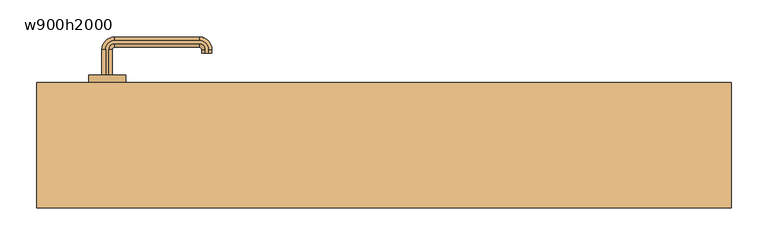
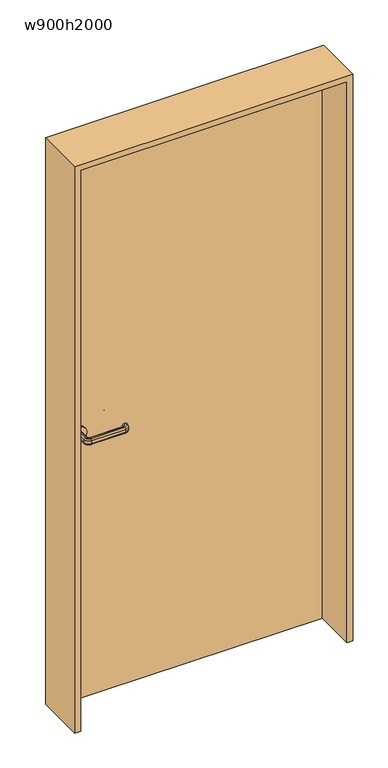
"""IFC4 building model written with IfcOpenShell, lengths in millimetres: door geometry, 片開き : w900h2000."""

from ifc_helpers import new_model, si_unit, point, frame, frame_2d, origin, origin_with_axes, place, context, project, spatial, polyline, circle_curve, ellipse_curve, trimmed, segment, composite_curve, outline, extrude, source, transform, mapped, element, save
from ifc_brep_helpers import plane_surface, cylinder_surface, revolved_surface, advanced_brep


def w900h2000_806be6ba(model_context):
    return source(origin(), model_context, "Body", "SolidModel", [
        advanced_brep(
        [(-377.0, 95.0, 960.0), (-382.0, 95.0, 955.0), (-382.0, 95.0, 945.0477623), (-377.0, 95.0, 940.0477623), (-373.0, 95.0, 940.0477623), (-368.0, 95.0, 945.0477623), (-368.0, 95.0, 955.0), (-373.0, 95.0, 960.0), (-377.0, 130.0, 960.0), (-382.0, 130.0, 955.0), (-382.0, 130.0, 945.0477623), (-377.0, 130.0, 940.0477623), (-365.0, 142.0, 940.0477623), (-250.0, 142.0, 940.0477623), (-238.0, 130.0, 940.0477623), (-238.0, 125.0, 940.0477623), (-242.0, 125.0, 940.0477623), (-242.0, 130.0, 940.0477623), (-250.0, 138.0, 940.0477623), (-365.0, 138.0, 940.0477623), (-373.0, 130.0, 940.0477623), (-368.0, 130.0, 945.0477623), (-368.0, 130.0, 955.0), (-373.0, 130.0, 960.0), (-365.0, 138.0, 960.0), (-250.0, 138.0, 960.0), (-242.0, 130.0, 960.0), (-242.0, 125.0, 960.0), (-238.0, 125.0, 960.0), (-238.0, 130.0, 960.0), (-250.0, 142.0, 960.0), (-365.0, 142.0, 960.0), (-365.0, 147.0, 955.0), (-365.0, 147.0, 945.0477623), (-365.0, 133.0, 945.0477623), (-365.0, 133.0, 955.0), (-250.0, 147.0, 955.0), (-250.0, 147.0, 945.0477623), (-250.0, 133.0, 945.0477623), (-250.0, 133.0, 955.0), (-233.0, 130.0, 955.0), (-233.0, 130.0, 945.0477623), (-247.0, 130.0, 945.0477623), (-247.0, 130.0, 955.0), (-247.0, 125.0, 955.0), (-247.0, 125.0, 945.0477623), (-233.0, 125.0, 945.0477623), (-233.0, 125.0, 955.0)],
        [
            (0, 1, circle_curve(frame((-377.0, 95.0, 955.0), z_axis=(0.0, -1.0, 0.0), x_axis=(-1.0, 0.0, 0.0)), 5.0)),
            (1, 2),
            (2, 3, circle_curve(frame((-377.0, 95.0, 945.0477623), z_axis=(0.0, -1.0, 0.0), x_axis=(-1.0, 0.0, 0.0)), 5.0)),
            (3, 4),
            (4, 5, circle_curve(frame((-373.0, 95.0, 945.0477623), z_axis=(0.0, -1.0, 0.0), x_axis=(-1.0, 0.0, 0.0)), 5.0)),
            (5, 6),
            (6, 7, circle_curve(frame((-373.0, 95.0, 955.0), z_axis=(0.0, -1.0, 0.0), x_axis=(-1.0, 0.0, 0.0)), 5.0)),
            (7, 0),
            (0, 8),
            (8, 9, circle_curve(frame((-377.0, 130.0, 955.0), z_axis=(0.0, -1.0, 0.0), x_axis=(-1.0, 0.0, 0.0)), 5.0)),
            (9, 1),
            (9, 10),
            (10, 2),
            (10, 11, circle_curve(frame((-377.0, 130.0, 945.0477623), z_axis=(0.0, -1.0, 0.0), x_axis=(-1.0, 0.0, 0.0)), 5.0)),
            (11, 3),
            (11, 12, circle_curve(frame((-365.0, 130.0, 940.0477623), z_axis=(0.0, 0.0, -1.0), x_axis=(-1.0, 0.0, 0.0)), 12.0)),
            (12, 13),
            (13, 14, circle_curve(frame((-250.0, 130.0, 940.0477623), z_axis=(0.0, 0.0, -1.0), x_axis=(0.0, 1.0, 0.0)), 12.0)),
            (14, 15),
            (15, 16),
            (16, 17),
            (17, 18, circle_curve(frame((-250.0, 130.0, 940.0477623), z_axis=(0.0, 0.0, 1.0), x_axis=(0.0, 1.0, 0.0)), 8.0)),
            (18, 19),
            (19, 20, circle_curve(frame((-365.0, 130.0, 940.0477623), z_axis=(0.0, 0.0, 1.0), x_axis=(-1.0, 0.0, 0.0)), 8.0)),
            (20, 4),
            (20, 21, circle_curve(frame((-373.0, 130.0, 945.0477623), z_axis=(0.0, -1.0, 0.0), x_axis=(-1.0, 0.0, 0.0)), 5.0)),
            (21, 5),
            (21, 22),
            (22, 6),
            (22, 23, circle_curve(frame((-373.0, 130.0, 955.0), z_axis=(0.0, -1.0, 0.0), x_axis=(-1.0, 0.0, 0.0)), 5.0)),
            (23, 7),
            (23, 24, circle_curve(frame((-365.0, 130.0, 960.0), z_axis=(0.0, 0.0, -1.0), x_axis=(-1.0, 0.0, 0.0)), 8.0)),
            (24, 25),
            (25, 26, circle_curve(frame((-250.0, 130.0, 960.0), z_axis=(0.0, 0.0, -1.0), x_axis=(0.0, 1.0, 0.0)), 8.0)),
            (26, 27),
            (27, 28),
            (28, 29),
            (29, 30, circle_curve(frame((-250.0, 130.0, 960.0), z_axis=(0.0, 0.0, 1.0), x_axis=(0.0, 1.0, 0.0)), 12.0)),
            (30, 31),
            (31, 8, circle_curve(frame((-365.0, 130.0, 960.0), z_axis=(0.0, 0.0, 1.0), x_axis=(-1.0, 0.0, 0.0)), 12.0)),
            (32, 9, circle_curve(frame((-365.0, 130.0, 955.0), z_axis=(0.0, 0.0, 1.0), x_axis=(-1.0, 0.0, 0.0)), 17.0)),
            (31, 32, circle_curve(frame((-365.0, 142.0, 955.0), z_axis=(-1.0, 0.0, 0.0), x_axis=(0.0, 1.0, 0.0)), 5.0)),
            (33, 10, circle_curve(frame((-365.0, 130.0, 945.0477623), z_axis=(0.0, 0.0, 1.0), x_axis=(-1.0, 0.0, 0.0)), 17.0)),
            (32, 33),
            (33, 12, circle_curve(frame((-365.0, 142.0, 945.0477623), z_axis=(-1.0, 0.0, 0.0), x_axis=(0.0, 1.0, 0.0)), 5.0)),
            (34, 21, circle_curve(frame((-365.0, 130.0, 945.0477623), z_axis=(0.0, 0.0, 1.0), x_axis=(-1.0, 0.0, 0.0)), 3.0)),
            (19, 34, circle_curve(frame((-365.0, 138.0, 945.0477623), z_axis=(-1.0, 0.0, 0.0), x_axis=(0.0, 1.0, 0.0)), 5.0)),
            (35, 22, circle_curve(frame((-365.0, 130.0, 955.0), z_axis=(0.0, 0.0, 1.0), x_axis=(-1.0, 0.0, 0.0)), 3.0)),
            (34, 35),
            (35, 24, circle_curve(frame((-365.0, 138.0, 955.0), z_axis=(-1.0, 0.0, 0.0), x_axis=(0.0, 1.0, 0.0)), 5.0)),
            (30, 36, circle_curve(frame((-250.0, 142.0, 955.0), z_axis=(-1.0, 0.0, 0.0), x_axis=(0.0, 1.0, 0.0)), 5.0)),
            (36, 32),
            (36, 37),
            (37, 33),
            (37, 13, circle_curve(frame((-250.0, 142.0, 945.0477623), z_axis=(-1.0, 0.0, 0.0), x_axis=(0.0, 1.0, 0.0)), 5.0)),
            (18, 38, circle_curve(frame((-250.0, 138.0, 945.0477623), z_axis=(-1.0, 0.0, 0.0), x_axis=(0.0, 1.0, 0.0)), 5.0)),
            (38, 34),
            (38, 39),
            (39, 35),
            (39, 25, circle_curve(frame((-250.0, 138.0, 955.0), z_axis=(-1.0, 0.0, 0.0), x_axis=(0.0, 1.0, 0.0)), 5.0)),
            (40, 36, circle_curve(frame((-250.0, 130.0, 955.0), z_axis=(0.0, 0.0, 1.0), x_axis=(0.0, 1.0, 0.0)), 17.0)),
            (29, 40, circle_curve(frame((-238.0, 130.0, 955.0), z_axis=(0.0, 1.0, 0.0), x_axis=(1.0, 0.0, 0.0)), 5.0)),
            (41, 37, circle_curve(frame((-250.0, 130.0, 945.0477623), z_axis=(0.0, 0.0, 1.0), x_axis=(0.0, 1.0, 0.0)), 17.0)),
            (40, 41),
            (41, 14, circle_curve(frame((-238.0, 130.0, 945.0477623), z_axis=(0.0, 1.0, 0.0), x_axis=(1.0, 0.0, 0.0)), 5.0)),
            (42, 38, circle_curve(frame((-250.0, 130.0, 945.0477623), z_axis=(0.0, 0.0, 1.0), x_axis=(0.0, 1.0, 0.0)), 3.0)),
            (17, 42, circle_curve(frame((-242.0, 130.0, 945.0477623), z_axis=(0.0, 1.0, 0.0), x_axis=(1.0, 0.0, 0.0)), 5.0)),
            (43, 39, circle_curve(frame((-250.0, 130.0, 955.0), z_axis=(0.0, 0.0, 1.0), x_axis=(0.0, 1.0, 0.0)), 3.0)),
            (42, 43),
            (43, 26, circle_curve(frame((-242.0, 130.0, 955.0), z_axis=(0.0, 1.0, 0.0), x_axis=(1.0, 0.0, 0.0)), 5.0)),
            (27, 44, circle_curve(frame((-242.0, 125.0, 955.0), z_axis=(0.0, -1.0, 0.0), x_axis=(1.0, 0.0, 0.0)), 5.0)),
            (44, 45),
            (45, 16, circle_curve(frame((-242.0, 125.0, 945.0477623), z_axis=(0.0, -1.0, 0.0), x_axis=(1.0, 0.0, 0.0)), 5.0)),
            (15, 46, circle_curve(frame((-238.0, 125.0, 945.0477623), z_axis=(0.0, -1.0, 0.0), x_axis=(1.0, 0.0, 0.0)), 5.0)),
            (46, 47),
            (47, 28, circle_curve(frame((-238.0, 125.0, 955.0), z_axis=(0.0, -1.0, 0.0), x_axis=(1.0, 0.0, 0.0)), 5.0)),
            (47, 40),
            (46, 41),
            (45, 42),
            (44, 43),
        ],
        [
            plane_surface(frame((-385.198039, 95.0, 950.0), z_axis=(0.0, -1.0, 0.0), x_axis=(0.0, 0.0, 1.0))),
            cylinder_surface(frame((-377.0, 95.0, 955.0), z_axis=(0.0, -1.0, 0.0), x_axis=(-1.0, 0.0, 0.0)), 5.0),
            plane_surface(frame((-382.0, 95.0, 955.0), z_axis=(-1.0, 0.0, 0.0), x_axis=(0.0, 1.0, 0.0))),
            cylinder_surface(frame((-377.0, 95.0, 945.0477623), z_axis=(0.0, -1.0, 0.0), x_axis=(-1.0, 0.0, 0.0)), 5.0),
            plane_surface(frame((-377.0, 95.0, 940.0477623), z_axis=(0.0, 0.0, -1.0), x_axis=(0.0, 1.0, 0.0))),
            cylinder_surface(frame((-373.0, 95.0, 945.0477623), z_axis=(0.0, -1.0, 0.0), x_axis=(-1.0, 0.0, 0.0)), 5.0),
            plane_surface(frame((-368.0, 95.0, 945.0477623), z_axis=(1.0, 0.0, 0.0), x_axis=(0.0, 1.0, 0.0))),
            cylinder_surface(frame((-373.0, 95.0, 955.0), z_axis=(0.0, -1.0, 0.0), x_axis=(-1.0, 0.0, 0.0)), 5.0),
            plane_surface(frame((-373.0, 95.0, 960.0), z_axis=(0.0, 0.0, 1.0), x_axis=(0.0, 1.0, 0.0))),
            revolved_surface(trimmed(ellipse_curve(frame((-377.0, 130.0, 955.0), z_axis=(0.0, -1.0, 0.0), x_axis=(-1.0, 0.0, 0.0)), 5.0, 5.0), [point((-377.0, 130.0, 960.0))], [point((-382.0, 130.0, 955.0))], True, "CARTESIAN"), (-365.0, 130.0, 950.0), (0.0, 0.0, -1.0)),
            cylinder_surface(frame((-365.0, 130.0, 950.0), z_axis=(0.0, 0.0, -1.0), x_axis=(-1.0, 0.0, 0.0)), 17.0),
            revolved_surface(trimmed(ellipse_curve(frame((-377.0, 130.0, 945.0477623), z_axis=(0.0, -1.0, 0.0), x_axis=(-1.0, 0.0, 0.0)), 5.0, 5.0), [point((-382.0, 130.0, 945.0477623))], [point((-377.0, 130.0, 940.0477623))], True, "CARTESIAN"), (-365.0, 130.0, 950.0), (0.0, 0.0, -1.0)),
            revolved_surface(trimmed(ellipse_curve(frame((-373.0, 130.0, 945.0477623), z_axis=(0.0, -1.0, 0.0), x_axis=(-1.0, 0.0, 0.0)), 5.0, 5.0), [point((-373.0, 130.0, 940.0477623))], [point((-368.0, 130.0, 945.0477623))], True, "CARTESIAN"), (-365.0, 130.0, 950.0), (0.0, 0.0, -1.0)),
            revolved_surface(polyline([(-368.0, 130.0, 945.0477623), (-368.0, 130.0, 955.0)]), (-365.0, 130.0, 950.0), (0.0, 0.0, -1.0)),
            revolved_surface(trimmed(ellipse_curve(frame((-373.0, 130.0, 955.0), z_axis=(0.0, -1.0, 0.0), x_axis=(-1.0, 0.0, 0.0)), 5.0, 5.0), [point((-368.0, 130.0, 955.0))], [point((-373.0, 130.0, 960.0))], True, "CARTESIAN"), (-365.0, 130.0, 950.0), (0.0, 0.0, -1.0)),
            cylinder_surface(frame((-365.0, 142.0, 955.0), z_axis=(-1.0, 0.0, 0.0), x_axis=(0.0, 1.0, 0.0)), 5.0),
            plane_surface(frame((-365.0, 147.0, 955.0), z_axis=(0.0, 1.0, 0.0), x_axis=(1.0, 0.0, 0.0))),
            cylinder_surface(frame((-365.0, 142.0, 945.0477623), z_axis=(-1.0, 0.0, 0.0), x_axis=(0.0, 1.0, 0.0)), 5.0),
            cylinder_surface(frame((-365.0, 138.0, 945.0477623), z_axis=(-1.0, 0.0, 0.0), x_axis=(0.0, 1.0, 0.0)), 5.0),
            plane_surface(frame((-365.0, 133.0, 945.0477623), z_axis=(0.0, -1.0, 0.0), x_axis=(1.0, 0.0, 0.0))),
            cylinder_surface(frame((-365.0, 138.0, 955.0), z_axis=(-1.0, 0.0, 0.0), x_axis=(0.0, 1.0, 0.0)), 5.0),
            revolved_surface(trimmed(ellipse_curve(frame((-250.0, 142.0, 955.0), z_axis=(-1.0, 0.0, 0.0), x_axis=(0.0, 1.0, 0.0)), 5.0, 5.0), [point((-250.0, 142.0, 960.0))], [point((-250.0, 147.0, 955.0))], True, "CARTESIAN"), (-250.0, 130.0, 950.0), (0.0, 0.0, -1.0)),
            cylinder_surface(frame((-250.0, 130.0, 950.0), z_axis=(0.0, 0.0, -1.0), x_axis=(0.0, 1.0, 0.0)), 17.0),
            revolved_surface(trimmed(ellipse_curve(frame((-250.0, 142.0, 945.0477623), z_axis=(-1.0, 0.0, 0.0), x_axis=(0.0, 1.0, 0.0)), 5.0, 5.0), [point((-250.0, 147.0, 945.0477623))], [point((-250.0, 142.0, 940.0477623))], True, "CARTESIAN"), (-250.0, 130.0, 950.0), (0.0, 0.0, -1.0)),
            revolved_surface(trimmed(ellipse_curve(frame((-250.0, 138.0, 945.0477623), z_axis=(-1.0, 0.0, 0.0), x_axis=(0.0, 1.0, 0.0)), 5.0, 5.0), [point((-250.0, 138.0, 940.0477623))], [point((-250.0, 133.0, 945.0477623))], True, "CARTESIAN"), (-250.0, 130.0, 950.0), (0.0, 0.0, -1.0)),
            revolved_surface(polyline([(-250.0, 133.0, 945.0477623), (-250.0, 133.0, 955.0)]), (-250.0, 130.0, 950.0), (0.0, 0.0, -1.0)),
            revolved_surface(trimmed(ellipse_curve(frame((-250.0, 138.0, 955.0), z_axis=(-1.0, 0.0, 0.0), x_axis=(0.0, 1.0, 0.0)), 5.0, 5.0), [point((-250.0, 133.0, 955.0))], [point((-250.0, 138.0, 960.0))], True, "CARTESIAN"), (-250.0, 130.0, 950.0), (0.0, 0.0, -1.0)),
            plane_surface(frame((-250.198039, 125.0, 950.0), z_axis=(0.0, -1.0, 0.0), x_axis=(0.0, 0.0, -1.0))),
            cylinder_surface(frame((-238.0, 130.0, 955.0), z_axis=(0.0, 1.0, 0.0), x_axis=(1.0, 0.0, 0.0)), 5.0),
            plane_surface(frame((-233.0, 130.0, 955.0), z_axis=(1.0, 0.0, 0.0), x_axis=(0.0, -1.0, 0.0))),
            cylinder_surface(frame((-238.0, 130.0, 945.0477623), z_axis=(0.0, 1.0, 0.0), x_axis=(1.0, 0.0, 0.0)), 5.0),
            cylinder_surface(frame((-242.0, 130.0, 945.0477623), z_axis=(0.0, 1.0, 0.0), x_axis=(1.0, 0.0, 0.0)), 5.0),
            plane_surface(frame((-247.0, 130.0, 945.0477623), z_axis=(-1.0, 0.0, 0.0), x_axis=(0.0, -1.0, 0.0))),
            cylinder_surface(frame((-242.0, 130.0, 955.0), z_axis=(0.0, 1.0, 0.0), x_axis=(1.0, 0.0, 0.0)), 5.0),
        ],
        [
            (0, [[1, 2, 3, 4, 5, 6, 7, 8]]),
            (1, [[-1, 9, 10, 11]]),
            (2, [[-2, -11, 12, 13]]),
            (3, [[-3, -13, 14, 15]]),
            (4, [[-4, -15, 16, 17, 18, 19, 20, 21, 22, 23, 24, 25]]),
            (5, [[-5, -25, 26, 27]]),
            (6, [[-6, -27, 28, 29]]),
            (7, [[-7, -29, 30, 31]]),
            (8, [[-8, -31, 32, 33, 34, 35, 36, 37, 38, 39, 40, -9]]),
            (9, [[41, -10, -40, 42]]),
            (10, [[43, -12, -41, 44]]),
            (11, [[-16, -14, -43, 45]]),
            (12, [[46, -26, -24, 47]]),
            (13, [[48, -28, -46, 49]]),
            (14, [[-32, -30, -48, 50]]),
            (15, [[-42, -39, 51, 52]]),
            (16, [[-44, -52, 53, 54]]),
            (17, [[-45, -54, 55, -17]]),
            (18, [[-47, -23, 56, 57]]),
            (19, [[-49, -57, 58, 59]]),
            (20, [[-50, -59, 60, -33]]),
            (21, [[61, -51, -38, 62]]),
            (22, [[63, -53, -61, 64]]),
            (23, [[-18, -55, -63, 65]]),
            (24, [[66, -56, -22, 67]]),
            (25, [[68, -58, -66, 69]]),
            (26, [[-34, -60, -68, 70]]),
            (27, [[-36, 71, 72, 73, -20, 74, 75, 76]]),
            (28, [[-62, -37, -76, 77]]),
            (29, [[-64, -77, -75, 78]]),
            (30, [[-65, -78, -74, -19]]),
            (31, [[-67, -21, -73, 79]]),
            (32, [[-69, -79, -72, 80]]),
            (33, [[-70, -80, -71, -35]]),
        ],
    ),
        advanced_brep(
        [(-373.0, 50.0, 940.0), (-377.0, 50.0, 940.0), (-382.0, 50.0, 945.0), (-382.0, 50.0, 955.0), (-377.0, 50.0, 960.0), (-373.0, 50.0, 960.0), (-368.0, 50.0, 955.0), (-368.0, 50.0, 945.0), (-373.0, 15.0, 940.0), (-365.0, 7.0, 940.0), (-250.0, 7.0, 940.0), (-242.0, 15.0, 940.0), (-242.0, 20.0, 940.0), (-238.0, 20.0, 940.0), (-238.0, 15.0, 940.0), (-250.0, 3.0, 940.0), (-365.0, 3.0, 940.0), (-377.0, 15.0, 940.0), (-382.0, 15.0, 945.0), (-382.0, 15.0, 955.0), (-377.0, 15.0, 960.0), (-365.0, 3.0, 960.0), (-250.0, 3.0, 960.0), (-238.0, 15.0, 960.0), (-238.0, 20.0, 960.0), (-242.0, 20.0, 960.0), (-242.0, 15.0, 960.0), (-250.0, 7.0, 960.0), (-365.0, 7.0, 960.0), (-373.0, 15.0, 960.0), (-368.0, 15.0, 955.0), (-368.0, 15.0, 945.0), (-365.0, -2.0, 945.0), (-365.0, -2.0, 955.0), (-365.0, 12.0, 955.0), (-365.0, 12.0, 945.0), (-250.0, -2.0, 945.0), (-250.0, -2.0, 955.0), (-250.0, 12.0, 955.0), (-250.0, 12.0, 945.0), (-233.0, 15.0, 945.0), (-233.0, 15.0, 955.0), (-247.0, 15.0, 955.0), (-247.0, 15.0, 945.0), (-247.0, 20.0, 945.0), (-247.0, 20.0, 955.0), (-233.0, 20.0, 955.0), (-233.0, 20.0, 945.0)],
        [
            (0, 1),
            (1, 2, circle_curve(frame((-377.0, 50.0, 945.0), z_axis=(0.0, 1.0, 0.0), x_axis=(1.0, 0.0, 0.0)), 5.0)),
            (2, 3),
            (3, 4, circle_curve(frame((-377.0, 50.0, 955.0), z_axis=(0.0, 1.0, 0.0), x_axis=(1.0, 0.0, 0.0)), 5.0)),
            (4, 5),
            (5, 6, circle_curve(frame((-373.0, 50.0, 955.0), z_axis=(0.0, 1.0, 0.0), x_axis=(1.0, 0.0, 0.0)), 5.0)),
            (6, 7),
            (7, 0, circle_curve(frame((-373.0, 50.0, 945.0), z_axis=(0.0, 1.0, 0.0), x_axis=(1.0, 0.0, 0.0)), 5.0)),
            (0, 8),
            (8, 9, circle_curve(frame((-365.0, 15.0, 940.0), z_axis=(0.0, 0.0, 1.0), x_axis=(-1.0, 0.0, 0.0)), 8.0)),
            (9, 10),
            (10, 11, circle_curve(frame((-250.0, 15.0, 940.0), z_axis=(0.0, 0.0, 1.0), x_axis=(0.0, -1.0, 0.0)), 8.0)),
            (11, 12),
            (12, 13),
            (13, 14),
            (14, 15, circle_curve(frame((-250.0, 15.0, 940.0), z_axis=(0.0, 0.0, -1.0), x_axis=(0.0, -1.0, 0.0)), 12.0)),
            (15, 16),
            (16, 17, circle_curve(frame((-365.0, 15.0, 940.0), z_axis=(0.0, 0.0, -1.0), x_axis=(-1.0, 0.0, 0.0)), 12.0)),
            (17, 1),
            (17, 18, circle_curve(frame((-377.0, 15.0, 945.0), z_axis=(0.0, 1.0, 0.0), x_axis=(1.0, 0.0, 0.0)), 5.0)),
            (18, 2),
            (18, 19),
            (19, 3),
            (19, 20, circle_curve(frame((-377.0, 15.0, 955.0), z_axis=(0.0, 1.0, 0.0), x_axis=(1.0, 0.0, 0.0)), 5.0)),
            (20, 4),
            (20, 21, circle_curve(frame((-365.0, 15.0, 960.0), z_axis=(0.0, 0.0, 1.0), x_axis=(-1.0, 0.0, 0.0)), 12.0)),
            (21, 22),
            (22, 23, circle_curve(frame((-250.0, 15.0, 960.0), z_axis=(0.0, 0.0, 1.0), x_axis=(0.0, -1.0, 0.0)), 12.0)),
            (23, 24),
            (24, 25),
            (25, 26),
            (26, 27, circle_curve(frame((-250.0, 15.0, 960.0), z_axis=(0.0, 0.0, -1.0), x_axis=(0.0, -1.0, 0.0)), 8.0)),
            (27, 28),
            (28, 29, circle_curve(frame((-365.0, 15.0, 960.0), z_axis=(0.0, 0.0, -1.0), x_axis=(-1.0, 0.0, 0.0)), 8.0)),
            (29, 5),
            (29, 30, circle_curve(frame((-373.0, 15.0, 955.0), z_axis=(0.0, 1.0, 0.0), x_axis=(1.0, 0.0, 0.0)), 5.0)),
            (30, 6),
            (30, 31),
            (31, 7),
            (31, 8, circle_curve(frame((-373.0, 15.0, 945.0), z_axis=(0.0, 1.0, 0.0), x_axis=(1.0, 0.0, 0.0)), 5.0)),
            (32, 18, circle_curve(frame((-365.0, 15.0, 945.0), z_axis=(0.0, 0.0, -1.0), x_axis=(-1.0, 0.0, 0.0)), 17.0)),
            (16, 32, circle_curve(frame((-365.0, 3.0, 945.0), z_axis=(-1.0, 0.0, 0.0), x_axis=(0.0, 1.0, 0.0)), 5.0)),
            (33, 19, circle_curve(frame((-365.0, 15.0, 955.0), z_axis=(0.0, 0.0, -1.0), x_axis=(-1.0, 0.0, 0.0)), 17.0)),
            (32, 33),
            (33, 21, circle_curve(frame((-365.0, 3.0, 955.0), z_axis=(-1.0, 0.0, 0.0), x_axis=(0.0, 1.0, 0.0)), 5.0)),
            (34, 30, circle_curve(frame((-365.0, 15.0, 955.0), z_axis=(0.0, 0.0, -1.0), x_axis=(-1.0, 0.0, 0.0)), 3.0)),
            (28, 34, circle_curve(frame((-365.0, 7.0, 955.0), z_axis=(-1.0, 0.0, 0.0), x_axis=(0.0, 1.0, 0.0)), 5.0)),
            (35, 31, circle_curve(frame((-365.0, 15.0, 945.0), z_axis=(0.0, 0.0, -1.0), x_axis=(-1.0, 0.0, 0.0)), 3.0)),
            (34, 35),
            (35, 9, circle_curve(frame((-365.0, 7.0, 945.0), z_axis=(-1.0, 0.0, 0.0), x_axis=(0.0, 1.0, 0.0)), 5.0)),
            (15, 36, circle_curve(frame((-250.0, 3.0, 945.0), z_axis=(-1.0, 0.0, 0.0), x_axis=(0.0, 1.0, 0.0)), 5.0)),
            (36, 32),
            (36, 37),
            (37, 33),
            (37, 22, circle_curve(frame((-250.0, 3.0, 955.0), z_axis=(-1.0, 0.0, 0.0), x_axis=(0.0, 1.0, 0.0)), 5.0)),
            (27, 38, circle_curve(frame((-250.0, 7.0, 955.0), z_axis=(-1.0, 0.0, 0.0), x_axis=(0.0, 1.0, 0.0)), 5.0)),
            (38, 34),
            (38, 39),
            (39, 35),
            (39, 10, circle_curve(frame((-250.0, 7.0, 945.0), z_axis=(-1.0, 0.0, 0.0), x_axis=(0.0, 1.0, 0.0)), 5.0)),
            (40, 36, circle_curve(frame((-250.0, 15.0, 945.0), z_axis=(0.0, 0.0, -1.0), x_axis=(0.0, -1.0, 0.0)), 17.0)),
            (14, 40, circle_curve(frame((-238.0, 15.0, 945.0), z_axis=(0.0, -1.0, 0.0), x_axis=(-1.0, 0.0, 0.0)), 5.0)),
            (41, 37, circle_curve(frame((-250.0, 15.0, 955.0), z_axis=(0.0, 0.0, -1.0), x_axis=(0.0, -1.0, 0.0)), 17.0)),
            (40, 41),
            (41, 23, circle_curve(frame((-238.0, 15.0, 955.0), z_axis=(0.0, -1.0, 0.0), x_axis=(-1.0, 0.0, 0.0)), 5.0)),
            (42, 38, circle_curve(frame((-250.0, 15.0, 955.0), z_axis=(0.0, 0.0, -1.0), x_axis=(0.0, -1.0, 0.0)), 3.0)),
            (26, 42, circle_curve(frame((-242.0, 15.0, 955.0), z_axis=(0.0, -1.0, 0.0), x_axis=(-1.0, 0.0, 0.0)), 5.0)),
            (43, 39, circle_curve(frame((-250.0, 15.0, 945.0), z_axis=(0.0, 0.0, -1.0), x_axis=(0.0, -1.0, 0.0)), 3.0)),
            (42, 43),
            (43, 11, circle_curve(frame((-242.0, 15.0, 945.0), z_axis=(0.0, -1.0, 0.0), x_axis=(-1.0, 0.0, 0.0)), 5.0)),
            (12, 44, circle_curve(frame((-242.0, 20.0, 945.0), z_axis=(0.0, 1.0, 0.0), x_axis=(-1.0, 0.0, 0.0)), 5.0)),
            (44, 45),
            (45, 25, circle_curve(frame((-242.0, 20.0, 955.0), z_axis=(0.0, 1.0, 0.0), x_axis=(-1.0, 0.0, 0.0)), 5.0)),
            (24, 46, circle_curve(frame((-238.0, 20.0, 955.0), z_axis=(0.0, 1.0, 0.0), x_axis=(-1.0, 0.0, 0.0)), 5.0)),
            (46, 47),
            (47, 13, circle_curve(frame((-238.0, 20.0, 945.0), z_axis=(0.0, 1.0, 0.0), x_axis=(-1.0, 0.0, 0.0)), 5.0)),
            (47, 40),
            (46, 41),
            (45, 42),
            (44, 43),
        ],
        [
            plane_surface(frame((-385.198039, 50.0, 950.0), z_axis=(0.0, 1.0, 0.0), x_axis=(0.0, 0.0, -1.0))),
            plane_surface(frame((-373.0, 50.0, 940.0), z_axis=(0.0, 0.0, -1.0), x_axis=(0.0, -1.0, 0.0))),
            cylinder_surface(frame((-377.0, 50.0, 945.0), z_axis=(0.0, 1.0, 0.0), x_axis=(1.0, 0.0, 0.0)), 5.0),
            plane_surface(frame((-382.0, 50.0, 945.0), z_axis=(-1.0, 0.0, 0.0), x_axis=(0.0, -1.0, 0.0))),
            cylinder_surface(frame((-377.0, 50.0, 955.0), z_axis=(0.0, 1.0, 0.0), x_axis=(1.0, 0.0, 0.0)), 5.0),
            plane_surface(frame((-377.0, 50.0, 960.0), z_axis=(0.0, 0.0, 1.0), x_axis=(0.0, -1.0, 0.0))),
            cylinder_surface(frame((-373.0, 50.0, 955.0), z_axis=(0.0, 1.0, 0.0), x_axis=(1.0, 0.0, 0.0)), 5.0),
            plane_surface(frame((-368.0, 50.0, 955.0), z_axis=(1.0, 0.0, 0.0), x_axis=(0.0, -1.0, 0.0))),
            cylinder_surface(frame((-373.0, 50.0, 945.0), z_axis=(0.0, 1.0, 0.0), x_axis=(1.0, 0.0, 0.0)), 5.0),
            revolved_surface(trimmed(ellipse_curve(frame((-377.0, 15.0, 945.0), z_axis=(0.0, 1.0, 0.0), x_axis=(1.0, 0.0, 0.0)), 5.0, 5.0), [point((-377.0, 15.0, 940.0))], [point((-382.0, 15.0, 945.0))], True, "CARTESIAN"), (-365.0, 15.0, 950.0), (0.0, 0.0, 1.0)),
            cylinder_surface(frame((-365.0, 15.0, 950.0), z_axis=(0.0, 0.0, 1.0), x_axis=(-1.0, 0.0, 0.0)), 17.0),
            revolved_surface(trimmed(ellipse_curve(frame((-377.0, 15.0, 955.0), z_axis=(0.0, 1.0, 0.0), x_axis=(1.0, 0.0, 0.0)), 5.0, 5.0), [point((-382.0, 15.0, 955.0))], [point((-377.0, 15.0, 960.0))], True, "CARTESIAN"), (-365.0, 15.0, 950.0), (0.0, 0.0, 1.0)),
            revolved_surface(trimmed(ellipse_curve(frame((-373.0, 15.0, 955.0), z_axis=(0.0, 1.0, 0.0), x_axis=(1.0, 0.0, 0.0)), 5.0, 5.0), [point((-373.0, 15.0, 960.0))], [point((-368.0, 15.0, 955.0))], True, "CARTESIAN"), (-365.0, 15.0, 950.0), (0.0, 0.0, 1.0)),
            revolved_surface(polyline([(-368.0, 15.0, 955.0), (-368.0, 15.0, 945.0)]), (-365.0, 15.0, 950.0), (0.0, 0.0, 1.0)),
            revolved_surface(trimmed(ellipse_curve(frame((-373.0, 15.0, 945.0), z_axis=(0.0, 1.0, 0.0), x_axis=(1.0, 0.0, 0.0)), 5.0, 5.0), [point((-368.0, 15.0, 945.0))], [point((-373.0, 15.0, 940.0))], True, "CARTESIAN"), (-365.0, 15.0, 950.0), (0.0, 0.0, 1.0)),
            cylinder_surface(frame((-365.0, 3.0, 945.0), z_axis=(-1.0, 0.0, 0.0), x_axis=(0.0, 1.0, 0.0)), 5.0),
            plane_surface(frame((-365.0, -2.0, 945.0), z_axis=(0.0, -1.0, 0.0), x_axis=(1.0, 0.0, 0.0))),
            cylinder_surface(frame((-365.0, 3.0, 955.0), z_axis=(-1.0, 0.0, 0.0), x_axis=(0.0, 1.0, 0.0)), 5.0),
            cylinder_surface(frame((-365.0, 7.0, 955.0), z_axis=(-1.0, 0.0, 0.0), x_axis=(0.0, 1.0, 0.0)), 5.0),
            plane_surface(frame((-365.0, 12.0, 955.0), z_axis=(0.0, 1.0, 0.0), x_axis=(1.0, 0.0, 0.0))),
            cylinder_surface(frame((-365.0, 7.0, 945.0), z_axis=(-1.0, 0.0, 0.0), x_axis=(0.0, 1.0, 0.0)), 5.0),
            revolved_surface(trimmed(ellipse_curve(frame((-250.0, 3.0, 945.0), z_axis=(-1.0, 0.0, 0.0), x_axis=(0.0, 1.0, 0.0)), 5.0, 5.0), [point((-250.0, 3.0, 940.0))], [point((-250.0, -2.0, 945.0))], True, "CARTESIAN"), (-250.0, 15.0, 950.0), (0.0, 0.0, 1.0)),
            cylinder_surface(frame((-250.0, 15.0, 950.0), z_axis=(0.0, 0.0, 1.0), x_axis=(0.0, -1.0, 0.0)), 17.0),
            revolved_surface(trimmed(ellipse_curve(frame((-250.0, 3.0, 955.0), z_axis=(-1.0, 0.0, 0.0), x_axis=(0.0, 1.0, 0.0)), 5.0, 5.0), [point((-250.0, -2.0, 955.0))], [point((-250.0, 3.0, 960.0))], True, "CARTESIAN"), (-250.0, 15.0, 950.0), (0.0, 0.0, 1.0)),
            revolved_surface(trimmed(ellipse_curve(frame((-250.0, 7.0, 955.0), z_axis=(-1.0, 0.0, 0.0), x_axis=(0.0, 1.0, 0.0)), 5.0, 5.0), [point((-250.0, 7.0, 960.0))], [point((-250.0, 12.0, 955.0))], True, "CARTESIAN"), (-250.0, 15.0, 950.0), (0.0, 0.0, 1.0)),
            revolved_surface(polyline([(-250.0, 12.0, 955.0), (-250.0, 12.0, 945.0)]), (-250.0, 15.0, 950.0), (0.0, 0.0, 1.0)),
            revolved_surface(trimmed(ellipse_curve(frame((-250.0, 7.0, 945.0), z_axis=(-1.0, 0.0, 0.0), x_axis=(0.0, 1.0, 0.0)), 5.0, 5.0), [point((-250.0, 12.0, 945.0))], [point((-250.0, 7.0, 940.0))], True, "CARTESIAN"), (-250.0, 15.0, 950.0), (0.0, 0.0, 1.0)),
            plane_surface(frame((-250.198039, 20.0, 950.0), z_axis=(0.0, 1.0, 0.0), x_axis=(0.0, 0.0, 1.0))),
            cylinder_surface(frame((-238.0, 15.0, 945.0), z_axis=(0.0, -1.0, 0.0), x_axis=(-1.0, 0.0, 0.0)), 5.0),
            plane_surface(frame((-233.0, 15.0, 945.0), z_axis=(1.0, 0.0, 0.0), x_axis=(0.0, 1.0, 0.0))),
            cylinder_surface(frame((-238.0, 15.0, 955.0), z_axis=(0.0, -1.0, 0.0), x_axis=(-1.0, 0.0, 0.0)), 5.0),
            cylinder_surface(frame((-242.0, 15.0, 955.0), z_axis=(0.0, -1.0, 0.0), x_axis=(-1.0, 0.0, 0.0)), 5.0),
            plane_surface(frame((-247.0, 15.0, 955.0), z_axis=(-1.0, 0.0, 0.0), x_axis=(0.0, 1.0, 0.0))),
            cylinder_surface(frame((-242.0, 15.0, 945.0), z_axis=(0.0, -1.0, 0.0), x_axis=(-1.0, 0.0, 0.0)), 5.0),
        ],
        [
            (0, [[1, 2, 3, 4, 5, 6, 7, 8]]),
            (1, [[-1, 9, 10, 11, 12, 13, 14, 15, 16, 17, 18, 19]]),
            (2, [[-2, -19, 20, 21]]),
            (3, [[-3, -21, 22, 23]]),
            (4, [[-4, -23, 24, 25]]),
            (5, [[-5, -25, 26, 27, 28, 29, 30, 31, 32, 33, 34, 35]]),
            (6, [[-6, -35, 36, 37]]),
            (7, [[-7, -37, 38, 39]]),
            (8, [[-8, -39, 40, -9]]),
            (9, [[41, -20, -18, 42]]),
            (10, [[43, -22, -41, 44]]),
            (11, [[-26, -24, -43, 45]]),
            (12, [[46, -36, -34, 47]]),
            (13, [[48, -38, -46, 49]]),
            (14, [[-10, -40, -48, 50]]),
            (15, [[-42, -17, 51, 52]]),
            (16, [[-44, -52, 53, 54]]),
            (17, [[-45, -54, 55, -27]]),
            (18, [[-47, -33, 56, 57]]),
            (19, [[-49, -57, 58, 59]]),
            (20, [[-50, -59, 60, -11]]),
            (21, [[61, -51, -16, 62]]),
            (22, [[63, -53, -61, 64]]),
            (23, [[-28, -55, -63, 65]]),
            (24, [[66, -56, -32, 67]]),
            (25, [[68, -58, -66, 69]]),
            (26, [[-12, -60, -68, 70]]),
            (27, [[71, 72, 73, -30, 74, 75, 76, -14]]),
            (28, [[-62, -15, -76, 77]]),
            (29, [[-64, -77, -75, 78]]),
            (30, [[-65, -78, -74, -29]]),
            (31, [[-67, -31, -73, 79]]),
            (32, [[-69, -79, -72, 80]]),
            (33, [[-70, -80, -71, -13]]),
        ],
    ),
        extrude(outline(composite_curve([segment(trimmed(circle_curve(frame_2d((950.0, -375.0)), 25.0), [point((950.0, -400.0))], [point((950.0, -350.0))], False, "CARTESIAN"), True, "CONTINUOUS"), segment(trimmed(circle_curve(frame_2d((950.0, -375.0)), 25.0), [point((950.0, -350.0))], [point((950.0, -400.0))], False, "CARTESIAN"), True, "CONTINUOUS")], self_intersect=False)), frame((0.0, 85.0, 0.0), z_axis=(0.0, 1.0, 0.0), x_axis=(0.0, 0.0, 1.0)), (0.0, 0.0, 1.0), 10.0),
        extrude(outline(composite_curve([segment(trimmed(circle_curve(frame_2d((950.0, -375.0)), 25.0), [point((950.0, -400.0))], [point((950.0, -350.0))], False, "CARTESIAN"), True, "CONTINUOUS"), segment(trimmed(circle_curve(frame_2d((950.0, -375.0)), 25.0), [point((950.0, -350.0))], [point((950.0, -400.0))], False, "CARTESIAN"), True, "CONTINUOUS")], self_intersect=False)), frame((0.0, 50.0, 0.0), z_axis=(0.0, 1.0, 0.0), x_axis=(0.0, 0.0, 1.0)), (0.0, 0.0, 1.0), 10.0),
        extrude(outline(polyline([(2020.0, -470.0), (0.0, -470.0), (0.0, -450.0), (2000.0, -450.0), (2000.0, 450.0), (0.0, 450.0), (0.0, 470.0), (2020.0, 470.0), (2020.0, -470.0)])), frame((0.0, -85.0, 0.0), z_axis=(0.0, 1.0, 0.0), x_axis=(0.0, 0.0, 1.0)), (0.0, 0.0, 1.0), 170.0),
        extrude(outline(polyline([(450.0, 60.0), (-450.0, 60.0), (-450.0, 85.0), (450.0, 85.0), (450.0, 60.0)])), origin_with_axes(), (0.0, 0.0, 1.0), 2000.0),
    ])


if __name__ == "__main__":
    model = new_model("IFC4")
    model_context = context("Model", 3, world=origin())
    ifc_project = project(units=[si_unit("LENGTHUNIT", "METRE", prefix="MILLI")], contexts=[model_context])
    site = spatial("IfcSite", under=ifc_project)
    building = spatial("IfcBuilding", under=site)
    placement = place(None, origin())
    w900h2000_shape = w900h2000_806be6ba(model_context)
    element("IfcDoor", 1, ObjectType="片開き : w900h2000", at=placement, inside=building, context=model_context, shape_type="MappedRepresentation", body=[
        mapped(w900h2000_shape, transform((0.0, 0.0, 0.0), x_axis=(1.0, 0.0, 0.0), y_axis=(0.0, 1.0, 0.0), z_axis=(0.0, 0.0, 1.0))),
    ])
    save(model, "model.ifc")

# Revit data of these elements
# Type "片開き : w900h2000"
#   Construction Type Id = "MDOOR"
#   Analytic Construction = "メタル"
#   Type Mark = "48"
#   Operation = "片側開き戸右"
#   Keynote = "08110.P2"
#   Visual Light Transmittance = 0
#   Solar Heat Gain Coefficient = 0
#   Heat Transfer Coefficient (U) = 3.7021 W/(m²·K)
#   高さ(中心) = 1000 mm
#   Height = 2000 mm
#   Thickness = 25 mm
#   ドア枠見附 = 20 mm
#   Width = 900 mm
#   取手取付け高さ = 950 mm
#   ドア枠ちり = 10 mm
#   Function = 0
#   ドア枠 [instance default] = 塗装ホワイト
#   ドア把手 [instance default] = メタル-ステンレス
#   ドア [instance default] = 塗装ホワイト
#   Wall Closure = (empty or 0)
# Element 1 (IfcDoor, "片開き : w900h2000")
#   Materials on its faces: "メタル-ステンレス", "塗装ホワイト"
# Materials
#   "塗装ホワイト": class "ペイント", colour RGB 249 249 249, transparency 0, Cost = 0
#   "メタル-ステンレス": class "メタル", colour RGB 247 247 247, transparency 0, Cost = 0
